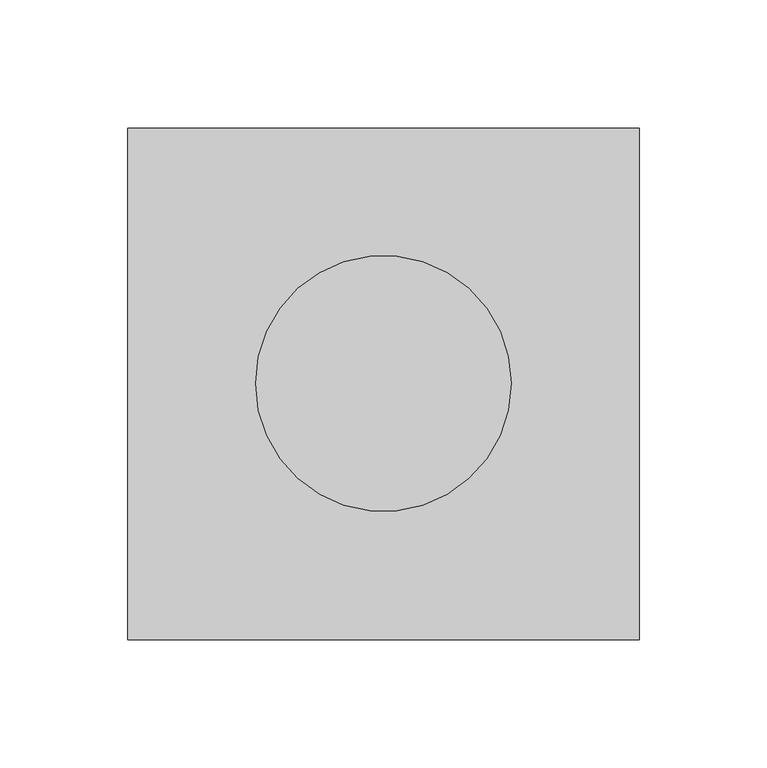
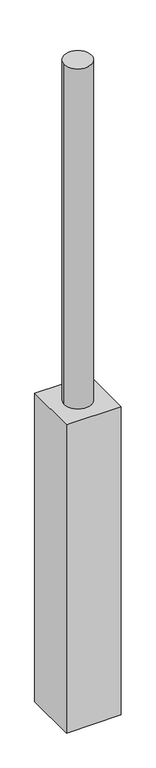
"""IFC4 building model written with IfcOpenShell, lengths in millimetres: proxy geometry, SDE4_ROOF_WEATHER VANE : SDE4_ROOF_WEATHER VANE."""

from ifc_helpers import new_model, si_unit, point, frame, frame_2d, origin, place, context, project, spatial, polyline, circle_curve, trimmed, segment, composite_curve, outline, extrude, source, transform, mapped, element, save


def generic_models_667129eb(model_context):
    return source(origin(), model_context, "Body", "SweptSolid", [
        extrude(outline(composite_curve([segment(trimmed(circle_curve(frame_2d((14487.4681025, 27100.0)), 50.0), [point((14437.4681025, 27100.0))], [point((14537.4681025, 27100.0))], False, "CARTESIAN"), True, "CONTINUOUS"), segment(trimmed(circle_curve(frame_2d((14487.4681025, 27100.0)), 50.0), [point((14537.4681025, 27100.0))], [point((14437.4681025, 27100.0))], False, "CARTESIAN"), True, "CONTINUOUS")], self_intersect=False)), frame((0.0, 0.0, 150233.133), z_axis=(0.0, 0.0, 1.0), x_axis=(1.0, 0.0, 0.0)), (0.0, 0.0, 1.0), 1312.0),
        extrude(outline(polyline([(14587.4681025, 27200.0), (14587.4681025, 27000.0), (14387.4681025, 27000.0), (14387.4681025, 27200.0), (14587.4681025, 27200.0)])), frame((0.0, 0.0, 149045.0), z_axis=(0.0, 0.0, 1.0), x_axis=(1.0, 0.0, 0.0)), (0.0, 0.0, 1.0), 1188.133),
    ])


if __name__ == "__main__":
    model = new_model("IFC4")
    model_context = context("Model", 3, world=origin())
    ifc_project = project(units=[si_unit("LENGTHUNIT", "METRE", prefix="MILLI")], contexts=[model_context])
    site = spatial("IfcSite", under=ifc_project)
    building = spatial("IfcBuilding", under=site)
    placement = place(None, origin())
    generic_models_shape = generic_models_667129eb(model_context)
    element("IfcBuildingElementProxy", 1, Name="SDE4_ROOF_WEATHER VANE : SDE4_ROOF_WEATHER VANE", ObjectType="SDE4_ROOF_WEATHER VANE : SDE4_ROOF_WEATHER VANE", at=placement, inside=building, context=model_context, shape_type="MappedRepresentation", body=[
        mapped(generic_models_shape, transform((0.0, 0.0, 0.0), x_axis=(1.0, 0.0, 0.0), y_axis=(0.0, 1.0, 0.0), z_axis=(0.0, 0.0, 1.0))),
    ])
    save(model, "model.ifc")
